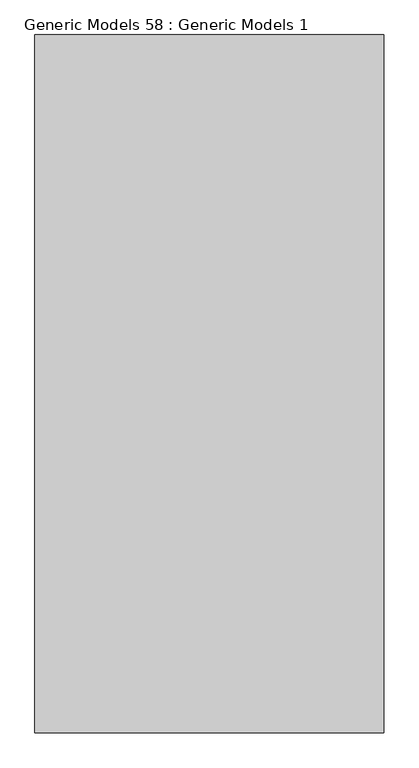
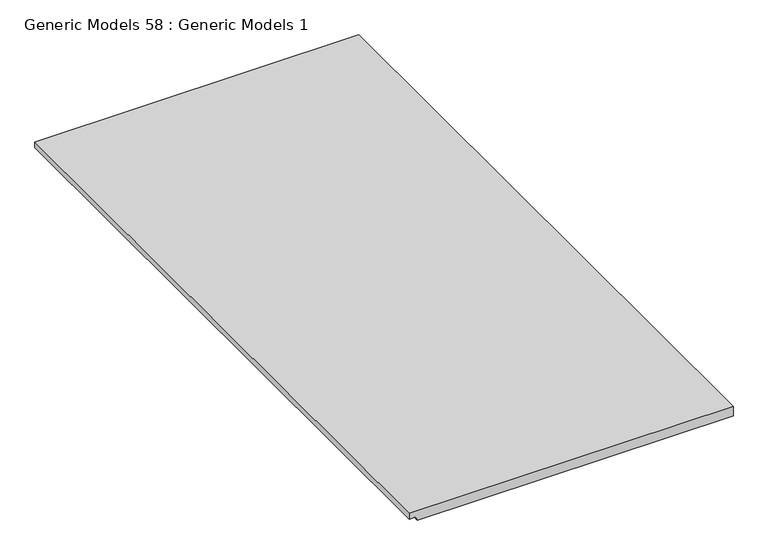
"""IFC4 building model written with IfcOpenShell, lengths in millimetres: proxy geometry, Generic Models 58 : Generic Models 1."""

from ifc_helpers import new_model, si_unit, frame, origin, place, context, project, spatial, polyline, outline, extrude, source, transform, mapped, element, save


def generic_models_58_generic_models_1_0ad20a8b(model_context):
    return source(origin(), model_context, "Body", "SweptSolid", [
        extrude(outline(polyline([(2253.330428, 49813.3451407), (2242.217928, 49813.3451407), (2242.217928, 49826.0451407), (2234.280428, 49828.9341545), (2234.280428, 50422.9451407), (2253.330428, 50422.9451407), (2253.330428, 49813.3451407)])), frame((0.0, 0.0, 0.0), z_axis=(0.0, 1.0, 0.0), x_axis=(0.0, 0.0, 1.0)), (0.0, 0.0, 1.0), 1219.2),
    ])


if __name__ == "__main__":
    model = new_model("IFC4")
    model_context = context("Model", 3, world=origin())
    ifc_project = project(units=[si_unit("LENGTHUNIT", "METRE", prefix="MILLI")], contexts=[model_context])
    site = spatial("IfcSite", under=ifc_project)
    building = spatial("IfcBuilding", under=site)
    placement = place(None, origin())
    generic_models_58_generic_models_1_shape = generic_models_58_generic_models_1_0ad20a8b(model_context)
    element("IfcBuildingElementProxy", 1, Name="Generic Models 58 : Generic Models 1", ObjectType="Generic Models 58 : Generic Models 1", at=placement, inside=building, context=model_context, shape_type="MappedRepresentation", body=[
        mapped(generic_models_58_generic_models_1_shape, transform((0.0, 0.0, 0.0), x_axis=(1.0, 0.0, 0.0), y_axis=(0.0, 1.0, 0.0), z_axis=(0.0, 0.0, 1.0))),
    ])
    save(model, "model.ifc")

# Revit data of these elements
# Element 1 (IfcBuildingElementProxy, "Generic Models 58 : Generic Models 1")
#   Materials on its faces: "CEILING AS SCHEDULED"
# Materials
#   "CEILING AS SCHEDULED": class "Generic", colour RGB 255 255 255, transparency 0, Cost = 0
